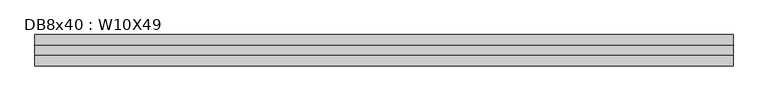
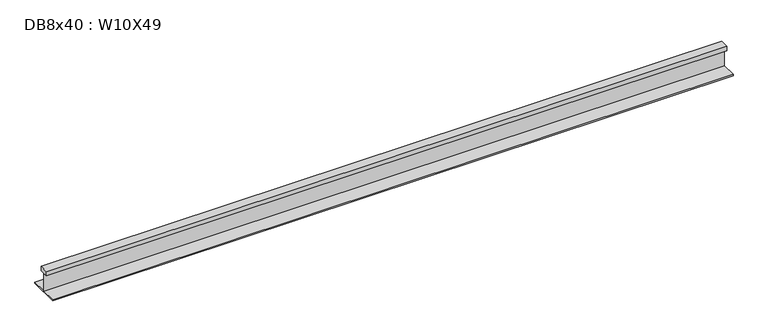
"""IFC4 building model written with IfcOpenShell, lengths in millimetres: beam geometry, DB8x40 : W10X49."""

from ifc_helpers import new_model, si_unit, frame, origin, place, context, project, spatial, polyline, outline, extrude, source, transform, mapped, element, save


def db8x40_w10x49_e545ec78(model_context):
    return source(origin(), model_context, "Body", "SweptSolid", [
        extrude(outline(polyline([(38.1, 144.3355), (38.1, 106.2355), (2.921, 106.2355), (2.921, -49.53), (127.0, -49.53), (127.0, -59.182), (-127.0, -59.182), (-127.0, -49.53), (-2.921, -49.53), (-2.921, 106.2355), (-38.1, 106.2355), (-38.1, 144.3355), (38.1, 144.3355)])), frame((-2902.2120761, 0.0, 0.0), z_axis=(1.0, 0.0, 0.0), x_axis=(0.0, 1.0, 0.0)), (0.0, 0.0, 1.0), 5668.0300658),
    ])


if __name__ == "__main__":
    model = new_model("IFC4")
    model_context = context("Model", 3, world=origin())
    ifc_project = project(units=[si_unit("LENGTHUNIT", "METRE", prefix="MILLI")], contexts=[model_context])
    site = spatial("IfcSite", under=ifc_project)
    building = spatial("IfcBuilding", under=site)
    placement = place(None, origin())
    db8x40_w10x49_shape = db8x40_w10x49_e545ec78(model_context)
    element("IfcBeam", 1, ObjectType="DB8x40 : W10X49", at=placement, inside=building, context=model_context, shape_type="MappedRepresentation", body=[
        mapped(db8x40_w10x49_shape, transform((0.0, 0.0, 0.0), x_axis=(1.0, 0.0, 0.0), y_axis=(0.0, 1.0, 0.0), z_axis=(0.0, 0.0, 1.0))),
    ])
    save(model, "model.ifc")

# Revit data of these elements
# Type "DB8x40 : W10X49"
#   Assembly Code = "B10"
#   W = 53
#   Length [instance default] = 5' - 0"
#   bf = 0' - 10"
#   d = 1' - 0.1"
#   k = 0' - 1 3/8"
#   k2 = 0' - 0.8"
#   tf = 0' - 0.575"
#   tw = 0' - 0.345"
#   A = 0.108333 SF
#   Structural Material [instance default] = Steel ASTM A992
# Element 1 (IfcBeam, "DB8x40 : W10X49")
#   Materials on its faces: "Steel ASTM A992"
# Materials
#   "Steel ASTM A992": class "Metal", colour RGB 199 199 199, transparency 0, Description = "Structural steel 50ksi", Cost = 0
